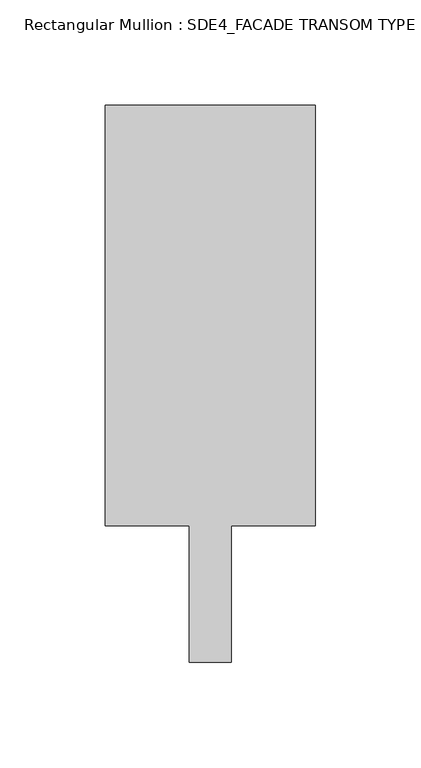
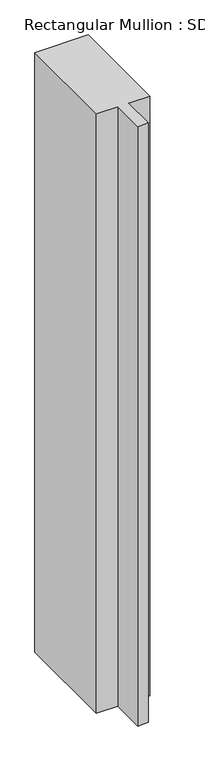
"""IFC4 building model written with IfcOpenShell, lengths in millimetres: member geometry, Rectangular Mullion : SDE4_FACADE TRANSOM TYPE 2."""

from ifc_helpers import new_model, si_unit, frame, origin, place, context, project, spatial, polyline, outline, extrude, source, transform, mapped, element, save


def rectangular_mullion_sde4_facade_transom_type_2_0ce523c0(model_context):
    return source(origin(), model_context, "Body", "SweptSolid", [
        extrude(outline(polyline([(50.0, 132.5), (50.0, -67.5), (10.0, -67.5), (10.0, -132.5), (-10.0, -132.5), (-10.0, -67.5), (-50.0, -67.5), (-50.0, 132.5), (50.0, 132.5)])), frame((0.0, 0.0, -1189.0000001), z_axis=(0.0, 0.0, 1.0), x_axis=(1.0, 0.0, 0.0)), (0.0, 0.0, 1.0), 1189.0000001),
    ])


if __name__ == "__main__":
    model = new_model("IFC4")
    model_context = context("Model", 3, world=origin())
    ifc_project = project(units=[si_unit("LENGTHUNIT", "METRE", prefix="MILLI")], contexts=[model_context])
    site = spatial("IfcSite", under=ifc_project)
    building = spatial("IfcBuilding", under=site)
    placement = place(None, origin())
    rectangular_mullion_sde4_facade_transom_type_2_shape = rectangular_mullion_sde4_facade_transom_type_2_0ce523c0(model_context)
    element("IfcMember", 1, ObjectType="Rectangular Mullion : SDE4_FACADE TRANSOM TYPE 2", at=placement, inside=building, context=model_context, shape_type="MappedRepresentation", body=[
        mapped(rectangular_mullion_sde4_facade_transom_type_2_shape, transform((0.0, 0.0, 0.0), x_axis=(1.0, 0.0, 0.0), y_axis=(0.0, 1.0, 0.0), z_axis=(0.0, 0.0, 1.0))),
    ])
    save(model, "model.ifc")

# Revit data of these elements
# Type "Rectangular Mullion : SDE4_FACADE TRANSOM TYPE 2"
#   built-in parameter 1007322 = 0.869423 (stored number, unit not read)
#   built-in parameter 1007321 = 0.164042 (stored number, unit not read)
#   built-in parameter 1007320 = 0.164042 (stored number, unit not read)
